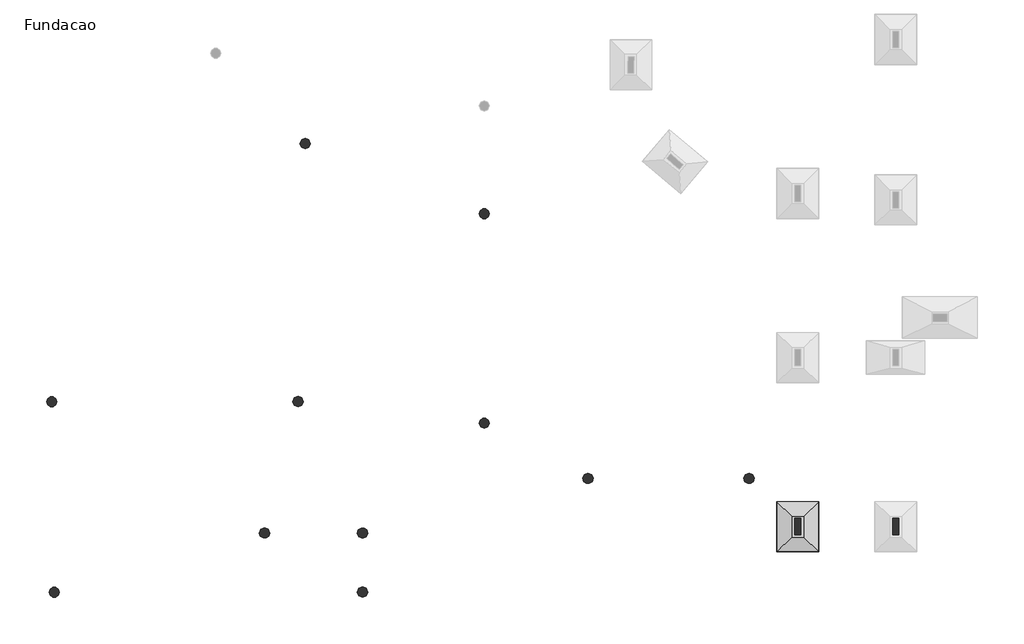
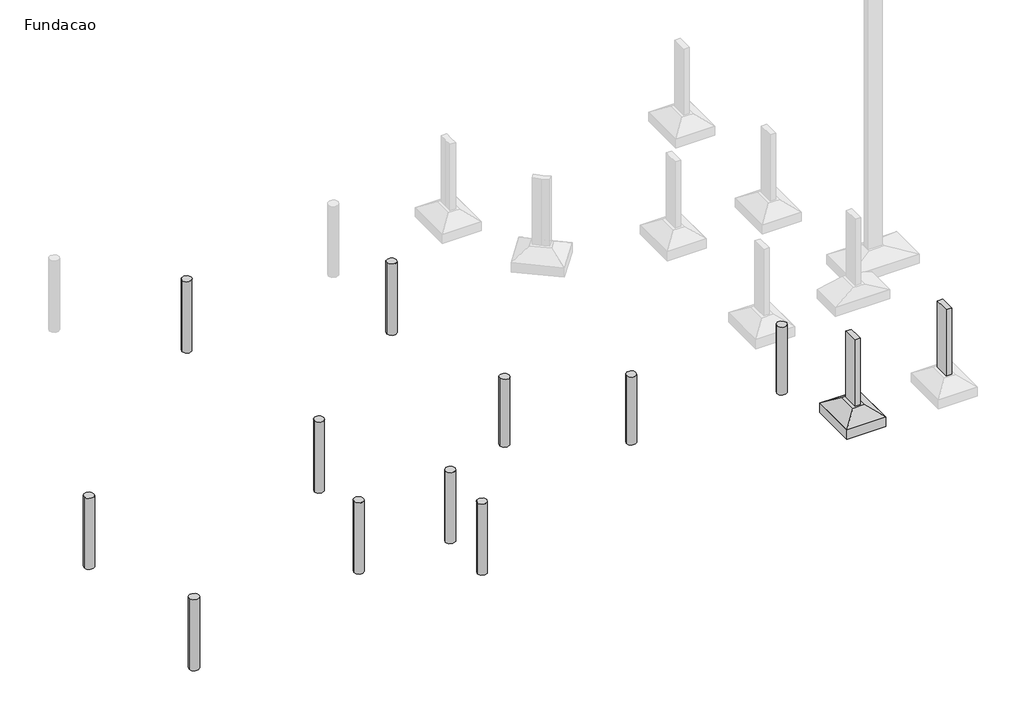
# One storey, part 1 of 2: 13 columns, 1 fastener.
"""IFC4 building model written with IfcOpenShell, lengths in millimetres."""

import ifcopenshell
import ifcopenshell.guid

model = None  # the IFC model being written
_history = None  # IfcOwnerHistory: only IFC2X3 demands one
_inside = {}  # id of a spatial element -> (the spatial element, [elements in it])
_under = {}  # id of a project, library or spatial element -> (it, [spatial elements below it])
_declared = {}  # id of a project -> (the project, [libraries it declares])
_typed = {}  # id of a type object -> (the type object, [elements of that type])
_made_of = {}  # id of a material, layer set ... -> (it, [elements and type objects made of it])


def new_model(schema):
    """Start an empty IFC model of exactly this schema.

    Asked for "IFC4X3", IfcOpenShell would pick the latest addendum, in which some entities
    have other attributes; the version numbers below select the first issue.
    IFC2X3 requires an IfcOwnerHistory on every rooted entity: one is made here for all.
    """
    global model, _history
    if schema == "IFC4X3":
        model = ifcopenshell.file(schema_version=(4, 3, 0, 0))
    else:
        model = ifcopenshell.file(schema=schema)
    _inside.clear()
    _under.clear()
    _declared.clear()
    _typed.clear()
    _made_of.clear()
    _history = None
    if model.schema == "IFC2X3":
        org = make("IfcOrganization", Name="unknown")
        user = make(
            "IfcPersonAndOrganization",
            ThePerson=make("IfcPerson", FamilyName="unknown"),
            TheOrganization=org,
        )
        app = make(
            "IfcApplication",
            ApplicationDeveloper=org,
            Version="unknown",
            ApplicationFullName="unknown",
            ApplicationIdentifier="unknown",
        )
        _history = make(
            "IfcOwnerHistory",
            OwningUser=user,
            OwningApplication=app,
            ChangeAction="ADDED",
            CreationDate=0,
        )
    return model


def make(cls, **values):
    """One entity of the class cls with the attributes given. An attribute that is None is left unset."""
    return model.create_entity(
        cls, **{name: value for name, value in values.items() if value is not None}
    )


def rooted(cls, **values):
    """An entity with a GlobalId (a new one), such as an element, a storey or a relation."""
    return make(cls, GlobalId=ifcopenshell.guid.new(), OwnerHistory=_history, **values)


def si_unit(unit_type, name, prefix=None):
    """IfcSIUnit, for example si_unit("LENGTHUNIT", "METRE", prefix="MILLI")."""
    return make("IfcSIUnit", UnitType=unit_type, Prefix=prefix, Name=name)


def assignment(units):
    """IfcUnitAssignment: the units of a project."""
    return None if units is None else make("IfcUnitAssignment", Units=units)


def point(xyz):
    """IfcCartesianPoint."""
    return None if xyz is None else make("IfcCartesianPoint", Coordinates=xyz)


def direction(xyz):
    """IfcDirection."""
    return None if xyz is None else make("IfcDirection", DirectionRatios=xyz)


def frame(location, z_axis=None, x_axis=None):
    """IfcAxis2Placement3D, a coordinate frame: its origin and axes. An axis left out is left unset."""
    return make(
        "IfcAxis2Placement3D",
        Location=point(location),
        Axis=direction(z_axis),
        RefDirection=direction(x_axis),
    )


def origin():
    """The frame at (0, 0, 0) with its axes left unset."""
    return frame((0.0, 0.0, 0.0))


def place(relative_to, where):
    """IfcLocalPlacement: puts the frame where relative to a parent placement (None: the world)."""
    return make(
        "IfcLocalPlacement", PlacementRelTo=relative_to, RelativePlacement=where
    )


def context(
    kind, dimensions, precision=None, world=None, true_north=None, identifier=None
):
    """IfcGeometricRepresentationContext, for example the 3D "Model" context."""
    return make(
        "IfcGeometricRepresentationContext",
        ContextIdentifier=identifier,
        ContextType=kind,
        CoordinateSpaceDimension=dimensions,
        Precision=precision,
        WorldCoordinateSystem=world,
        TrueNorth=true_north,
    )


def project(units=None, contexts=None):
    """IfcProject with its units and contexts."""
    return rooted(
        "IfcProject",
        Name="project",
        RepresentationContexts=contexts,
        UnitsInContext=assignment(units),
    )


def spatial(cls, under=None, at=None, **own):
    """A site, building, storey or space (cls), placed at a placement, below another one or the project."""
    s = rooted(cls, ObjectPlacement=at, **own)
    if under is not None:
        _under.setdefault(under.id(), (under, []))[1].append(s)
    return s


def polyline(points):
    """IfcPolyline through the points."""
    return make("IfcPolyline", Points=[point(p) for p in points])


def circle_curve(where, radius):
    """IfcCircle in the frame where."""
    return make("IfcCircle", Position=where, Radius=radius)


def outline(outer, holes=None, kind="AREA"):
    """IfcArbitraryClosedProfileDef: a profile drawn as a closed curve; with holes, ...WithVoids."""
    if holes is None:
        return make("IfcArbitraryClosedProfileDef", ProfileType=kind, OuterCurve=outer)
    return make(
        "IfcArbitraryProfileDefWithVoids",
        ProfileType=kind,
        OuterCurve=outer,
        InnerCurves=holes,
    )


def extrude(swept, where, along, depth):
    """IfcExtrudedAreaSolid: the profile swept, set in the frame where, extruded along a direction by depth."""
    return make(
        "IfcExtrudedAreaSolid",
        SweptArea=swept,
        Position=where,
        ExtrudedDirection=direction(along),
        Depth=depth,
    )


def faces_of(points, faces, orient=None, outer=None):
    """IfcFace entities. A face is a list of loops; a loop is a list of indices into points, from 0.

    orient and outer hold one flag for each loop. By default every Orientation is true, the
    first loop of a face is its IfcFaceOuterBound and the others are IfcFaceBound.
    """
    made = []
    for i, loops in enumerate(faces):
        bounds = []
        for j, loop in enumerate(loops):
            is_outer = j == 0 if outer is None else outer[i][j]
            bounds.append(
                make(
                    "IfcFaceOuterBound" if is_outer else "IfcFaceBound",
                    Bound=make("IfcPolyLoop", Polygon=[points[k] for k in loop]),
                    Orientation=True if orient is None else orient[i][j],
                )
            )
        made.append(make("IfcFace", Bounds=bounds))
    return made


def faceted_brep(points, faces, orient=None, outer=None, voids=None):
    """IfcFacetedBrep: a solid bounded by flat faces; with voids (closed shells), ...WithVoids."""
    shared = [point(p) for p in points]
    hull = make("IfcClosedShell", CfsFaces=faces_of(shared, faces, orient, outer))
    if voids is None:
        return make("IfcFacetedBrep", Outer=hull)
    return make(
        "IfcFacetedBrepWithVoids",
        Outer=hull,
        Voids=[
            make(cls, CfsFaces=faces_of(shared, fs, o, b)) for cls, fs, o, b in voids
        ],
    )


def shape(context_of_items, identifier, shape_type, items):
    """IfcShapeRepresentation: the items that make up one representation, for example the "Body"."""
    return make(
        "IfcShapeRepresentation",
        ContextOfItems=context_of_items,
        RepresentationIdentifier=identifier,
        RepresentationType=shape_type,
        Items=items,
    )


def source(mapping_origin, context_of_items, identifier, shape_type, items):
    """IfcRepresentationMap: a shape defined once, which mapped items show again and again."""
    return make(
        "IfcRepresentationMap",
        MappingOrigin=mapping_origin,
        MappedRepresentation=shape(context_of_items, identifier, shape_type, items),
    )


def transform(
    local_origin,
    x_axis=None,
    y_axis=None,
    z_axis=None,
    scale=None,
    scale2=None,
    scale3=None,
    uniform=True,
):
    """IfcCartesianTransformationOperator3D, or its non-uniform kind. x_axis, y_axis, z_axis: its Axis1, 2, 3."""
    if uniform:
        return make(
            "IfcCartesianTransformationOperator3D",
            Axis1=direction(x_axis),
            Axis2=direction(y_axis),
            LocalOrigin=point(local_origin),
            Scale=scale,
            Axis3=direction(z_axis),
        )
    return make(
        "IfcCartesianTransformationOperator3DnonUniform",
        Axis1=direction(x_axis),
        Axis2=direction(y_axis),
        LocalOrigin=point(local_origin),
        Scale=scale,
        Axis3=direction(z_axis),
        Scale2=scale2,
        Scale3=scale3,
    )


def mapped(mapping_source, mapping_target):
    """IfcMappedItem: shows the shape of a source again, moved by a transform."""
    return make(
        "IfcMappedItem", MappingSource=mapping_source, MappingTarget=mapping_target
    )


def made_of(thing, what):
    """Note that an element or type object is made of a material, layer set ...; save() writes the relation."""
    if what is not None:
        _made_of.setdefault(what.id(), (what, []))[1].append(thing)
    return thing


def element(
    cls,
    number,
    at=None,
    inside=None,
    cuts=None,
    type_object=None,
    material=None,
    context=None,
    identifier="Body",
    shape_type=None,
    held_by="IfcProductDefinitionShape",
    body=None,
    shapes=None,
    **own,
):
    """One element of the class cls, such as IfcWall. Its Tag is "e" and its number.

    at: its placement. inside: the storey or other place that contains it. cuts: it is an
    opening in that element (IfcRelVoidsElement). A single representation is given by context,
    identifier, shape_type and body (its items); several are given by shapes. held_by: the class
    of the entity that holds the representations. save() writes the other relations.
    """
    e = rooted(cls, Tag="e%d" % number, ObjectPlacement=at, **own)
    if body is not None:
        shapes = [shape(context, identifier, shape_type, body)]
    if shapes is not None:
        e.Representation = make(held_by, Representations=shapes)
    if inside is not None:
        _inside.setdefault(inside.id(), (inside, []))[1].append(e)
    if cuts is not None:
        rooted(
            "IfcRelVoidsElement", RelatingBuildingElement=cuts, RelatedOpeningElement=e
        )
    if type_object is not None:
        _typed.setdefault(type_object.id(), (type_object, []))[1].append(e)
    return made_of(e, material)


def aggregate(whole, parts):
    """IfcRelAggregates: a whole, such as a stair, and the parts it consists of."""
    return rooted("IfcRelAggregates", RelatingObject=whole, RelatedObjects=parts)


def save(model, path):
    """Write the relations noted so far, then the file.

    IfcRelAggregates (storeys below a building ...), IfcRelContainedInSpatialStructure (elements
    in a storey), IfcRelDefinesByType, IfcRelAssociatesMaterial and IfcRelDeclares: one each for
    every whole, place, type object, material and project.
    """
    for whole, parts in _under.values():
        aggregate(whole, parts)
    for where, things in _inside.values():
        rooted(
            "IfcRelContainedInSpatialStructure",
            RelatedElements=things,
            RelatingStructure=where,
        )
    for kind, things in _typed.values():
        rooted("IfcRelDefinesByType", RelatedObjects=things, RelatingType=kind)
    for what, things in _made_of.values():
        rooted("IfcRelAssociatesMaterial", RelatedObjects=things, RelatingMaterial=what)
    for by, libraries in _declared.values():
        rooted("IfcRelDeclares", RelatingContext=by, RelatedDefinitions=libraries)
    model.write(path)


def plane_surface(at):
    """IfcPlane: the flat surface through the origin of the frame at, square to its z axis."""
    return make("IfcPlane", Position=at)


def cylinder_surface(at, radius):
    """IfcCylindricalSurface: all points at the distance radius from the z axis of the frame at."""
    return make("IfcCylindricalSurface", Position=at, Radius=radius)


def advanced_brep(points, edges, surfaces, faces):
    """IfcAdvancedBrep: a solid bounded by faces that lie on surfaces and meet in shared edges.

    An edge is (start, end): straight between two places in points (the first is 0);
    or (start, end, curve); or (start, end, curve, False) where it runs against its curve.
    A face is (place in surfaces, loops), or (place, loops, False) where it looks against
    its surface's normal. A loop lists edges by number (the first is 1), with a minus sign
    where the edge is run from its end to its start. The first loop is the outer one.
    """
    corners = [point(p) for p in points]
    vertices = [make("IfcVertexPoint", VertexGeometry=c) for c in corners]
    made = []
    for start, end, *more in edges:
        made.append(
            make(
                "IfcEdgeCurve",
                EdgeStart=vertices[start],
                EdgeEnd=vertices[end],
                EdgeGeometry=more[0] if more else make("IfcPolyline", Points=[corners[start], corners[end]]),
                SameSense=more[1] if len(more) > 1 else True,
            )
        )
    hull = []
    for where, loops, *sense in faces:
        bounds = []
        for j, loop in enumerate(loops):
            ring = [make("IfcOrientedEdge", EdgeElement=made[abs(k) - 1], Orientation=k > 0) for k in loop]
            bounds.append(
                make(
                    "IfcFaceOuterBound" if j == 0 else "IfcFaceBound",
                    Bound=make("IfcEdgeLoop", EdgeList=ring),
                    Orientation=True,
                )
            )
        hull.append(make("IfcAdvancedFace", Bounds=bounds, FaceSurface=surfaces[where], SameSense=sense[0] if sense else True))
    return make("IfcAdvancedBrep", Outer=make("IfcClosedShell", CfsFaces=hull))


def sps1_6b3be553(model_context):
    return source(origin(), model_context, "Body", "SolidModel", [
        faceted_brep([(-55.0, 50.0, 0.0), (-345.0, 50.0, 0.0), (-345.0, -450.0, 0.0), (-55.0, -450.0, 0.0), (300.0, 400.0, -250.0), (300.0, -800.0, -250.0), (-700.0, -800.0, -250.0), (-700.0, 400.0, -250.0)], [[[0, 1, 2, 3]], [[4, 5, 6, 7]], [[4, 7, 1, 0]], [[7, 6, 2, 1]], [[6, 5, 3, 2]], [[5, 4, 0, 3]]]),
        extrude(outline(polyline([(300.0, 400.0), (300.0, -800.0), (-700.0, -800.0), (-700.0, 400.0), (300.0, 400.0)])), frame((0.0, 0.0, -500.0), z_axis=(0.0, 0.0, 1.0), x_axis=(1.0, 0.0, 0.0)), (0.0, 0.0, 1.0), 250.0),
    ])


model = new_model("IFC4")

# Units and contexts
model_context = context("Model", 3, world=origin())
ifc_project = project(units=[si_unit("LENGTHUNIT", "METRE", prefix="MILLI")], contexts=[model_context])

# Site, building, storey
site = spatial("IfcSite", under=ifc_project)
building = spatial("IfcBuilding", under=site)
storey = spatial("IfcBuildingStorey", under=building, Name="Fundacao", Elevation=-1200.0)

# Columns
placement = place(None, origin())
element("IfcColumn", 1, ObjectType="TQS - Pilar circular : TQS - Pilar circular 25.0cm", at=placement, inside=storey, context=model_context, shape_type="AdvancedBrep", body=[
    advanced_brep(
    [(-3146.281307, -11048.5699847, -1500.0), (-2896.281307, -11048.5699847, -1500.0), (-3146.281307, -11048.5699847, 430.0), (-3102.521691, -10953.5699847, 430.0), (-2896.281307, -11048.5699847, 430.0), (-3102.521691, -11143.5699847, 430.0)],
    [
        (0, 1, circle_curve(frame((-3021.281307, -11048.5699847, -1500.0), z_axis=(0.0, 0.0, -1.0), x_axis=(1.0, 0.0, 0.0)), 125.0)),
        (1, 0, circle_curve(frame((-3021.281307, -11048.5699847, -1500.0), z_axis=(0.0, 0.0, -1.0), x_axis=(1.0, 0.0, 0.0)), 125.0)),
        (2, 3, circle_curve(frame((-3021.281307, -11048.5699847, 430.0), z_axis=(0.0, 0.0, -1.0), x_axis=(1.0, 0.0, 0.0)), 125.0)),
        (3, 4, circle_curve(frame((-3021.281307, -11048.5699847, 430.0), z_axis=(0.0, 0.0, -1.0), x_axis=(1.0, 0.0, 0.0)), 125.0)),
        (4, 1),
        (0, 2),
        (4, 5, circle_curve(frame((-3021.281307, -11048.5699847, 430.0), z_axis=(0.0, 0.0, -1.0), x_axis=(1.0, 0.0, 0.0)), 125.0)),
        (5, 2, circle_curve(frame((-3021.281307, -11048.5699847, 430.0), z_axis=(0.0, 0.0, -1.0), x_axis=(1.0, 0.0, 0.0)), 125.0)),
    ],
    [
        plane_surface(frame((-2896.281307, -11048.5699847, -1500.0), z_axis=(0.0, 0.0, -1.0), x_axis=(0.0, -1.0, 0.0))),
        cylinder_surface(frame((-3021.281307, -11048.5699847, -1500.0), z_axis=(0.0, 0.0, 1.0), x_axis=(1.0, 0.0, 0.0)), 125.0),
        plane_surface(frame((-2896.281307, -11048.5699847, 430.0), z_axis=(0.0, 0.0, 1.0), x_axis=(0.0, 1.0, 0.0))),
    ],
    [
        (0, [[1, 2]]),
        (1, [[3, 4, 5, -1, 6]]),
        (1, [[7, 8, -6, -2, -5]]),
        (2, [[-8, -7, -4, -3]]),
    ],
),
])
element("IfcColumn", 2, ObjectType="TQS - Pilar circular : TQS - Pilar circular 25.0cm", at=placement, inside=storey, context=model_context, shape_type="AdvancedBrep", body=[
    advanced_brep(
    [(-3146.281307, -9633.3699847, -1500.0), (-2896.281307, -9633.3699847, -1500.0), (-3146.281307, -9633.3699847, 430.0), (-3124.8428828, -9563.3699847, 430.0), (-2896.281307, -9633.3699847, 430.0), (-3124.8428828, -9703.3699847, 430.0)],
    [
        (0, 1, circle_curve(frame((-3021.281307, -9633.3699847, -1500.0), z_axis=(0.0, 0.0, -1.0), x_axis=(1.0, 0.0, 0.0)), 125.0)),
        (1, 0, circle_curve(frame((-3021.281307, -9633.3699847, -1500.0), z_axis=(0.0, 0.0, -1.0), x_axis=(1.0, 0.0, 0.0)), 125.0)),
        (2, 3, circle_curve(frame((-3021.281307, -9633.3699847, 430.0), z_axis=(0.0, 0.0, -1.0), x_axis=(1.0, 0.0, 0.0)), 125.0)),
        (3, 4, circle_curve(frame((-3021.281307, -9633.3699847, 430.0), z_axis=(0.0, 0.0, -1.0), x_axis=(1.0, 0.0, 0.0)), 125.0)),
        (4, 1),
        (0, 2),
        (4, 5, circle_curve(frame((-3021.281307, -9633.3699847, 430.0), z_axis=(0.0, 0.0, -1.0), x_axis=(1.0, 0.0, 0.0)), 125.0)),
        (5, 2, circle_curve(frame((-3021.281307, -9633.3699847, 430.0), z_axis=(0.0, 0.0, -1.0), x_axis=(1.0, 0.0, 0.0)), 125.0)),
    ],
    [
        plane_surface(frame((-2896.281307, -9633.3699847, -1500.0), z_axis=(0.0, 0.0, -1.0), x_axis=(0.0, -1.0, 0.0))),
        cylinder_surface(frame((-3021.281307, -9633.3699847, -1500.0), z_axis=(0.0, 0.0, 1.0), x_axis=(1.0, 0.0, 0.0)), 125.0),
        plane_surface(frame((-2896.281307, -9633.3699847, 430.0), z_axis=(0.0, 0.0, 1.0), x_axis=(0.0, 1.0, 0.0))),
    ],
    [
        (0, [[1, 2]]),
        (1, [[3, 4, 5, -1, 6]]),
        (1, [[7, 8, -6, -2, -5]]),
        (2, [[-8, -7, -4, -3]]),
    ],
),
])
element("IfcColumn", 3, ObjectType="TQS - Pilar circular : TQS - Pilar circular 25.0cm", at=placement, inside=storey, context=model_context, shape_type="AdvancedBrep", body=[
    advanced_brep(
    [(-10536.281307, -11048.5699847, -1500.0), (-10286.281307, -11048.5699847, -1500.0), (-10536.281307, -11048.5699847, 430.0), (-10492.499945, -10953.5513927, 430.0), (-10401.3039585, -10923.9688109, 430.0), (-10330.0409229, -10953.5699847, 430.0), (-10286.281307, -11048.5699847, 430.0), (-10330.0409229, -11143.5699847, 430.0), (-10492.499945, -11143.5885767, 430.0)],
    [
        (0, 1, circle_curve(frame((-10411.281307, -11048.5699847, -1500.0), z_axis=(0.0, 0.0, -1.0), x_axis=(1.0, 0.0, 0.0)), 125.0)),
        (1, 0, circle_curve(frame((-10411.281307, -11048.5699847, -1500.0), z_axis=(0.0, 0.0, -1.0), x_axis=(1.0, 0.0, 0.0)), 125.0)),
        (2, 3, circle_curve(frame((-10411.281307, -11048.5699847, 430.0), z_axis=(0.0, 0.0, -1.0), x_axis=(1.0, 0.0, 0.0)), 125.0)),
        (3, 4, circle_curve(frame((-10411.281307, -11048.5699847, 430.0), z_axis=(0.0, 0.0, -1.0), x_axis=(1.0, 0.0, 0.0)), 125.0)),
        (4, 5, circle_curve(frame((-10411.281307, -11048.5699847, 430.0), z_axis=(0.0, 0.0, -1.0), x_axis=(1.0, 0.0, 0.0)), 125.0)),
        (5, 6, circle_curve(frame((-10411.281307, -11048.5699847, 430.0), z_axis=(0.0, 0.0, -1.0), x_axis=(1.0, 0.0, 0.0)), 125.0)),
        (6, 1),
        (0, 2),
        (6, 7, circle_curve(frame((-10411.281307, -11048.5699847, 430.0), z_axis=(0.0, 0.0, -1.0), x_axis=(1.0, 0.0, 0.0)), 125.0)),
        (7, 8, circle_curve(frame((-10411.281307, -11048.5699847, 430.0), z_axis=(0.0, 0.0, -1.0), x_axis=(1.0, 0.0, 0.0)), 125.0)),
        (8, 2, circle_curve(frame((-10411.281307, -11048.5699847, 430.0), z_axis=(0.0, 0.0, -1.0), x_axis=(1.0, 0.0, 0.0)), 125.0)),
    ],
    [
        plane_surface(frame((-10286.281307, -11048.5699847, -1500.0), z_axis=(0.0, 0.0, -1.0), x_axis=(0.0, -1.0, 0.0))),
        cylinder_surface(frame((-10411.281307, -11048.5699847, -1500.0), z_axis=(0.0, 0.0, 1.0), x_axis=(1.0, 0.0, 0.0)), 125.0),
        plane_surface(frame((-10286.281307, -11048.5699847, 430.0), z_axis=(0.0, 0.0, 1.0), x_axis=(0.0, 1.0, 0.0))),
    ],
    [
        (0, [[1, 2]]),
        (1, [[3, 4, 5, 6, 7, -1, 8]]),
        (1, [[9, 10, 11, -8, -2, -7]]),
        (2, [[-11, -10, -9, -6, -5, -4, -3]]),
    ],
),
])
element("IfcColumn", 4, ObjectType="TQS - Pilar circular : TQS - Pilar circular 25.0cm", at=placement, inside=storey, context=model_context, shape_type="AdvancedBrep", body=[
    advanced_brep(
    [(-4522.481307, -299.9062997, -1500.0), (-4272.481307, -299.9062997, -1500.0), (-4522.481307, -299.9062997, 430.0), (-4272.481307, -299.9062997, 430.0), (-4327.481307, -403.4678755, 430.0), (-4467.481307, -403.4678755, 430.0)],
    [
        (0, 1, circle_curve(frame((-4397.481307, -299.9062997, -1500.0), z_axis=(0.0, 0.0, -1.0), x_axis=(1.0, 0.0, 0.0)), 125.0)),
        (1, 0, circle_curve(frame((-4397.481307, -299.9062997, -1500.0), z_axis=(0.0, 0.0, -1.0), x_axis=(1.0, 0.0, 0.0)), 125.0)),
        (2, 3, circle_curve(frame((-4397.481307, -299.9062997, 430.0), z_axis=(0.0, 0.0, -1.0), x_axis=(1.0, 0.0, 0.0)), 125.0)),
        (3, 1),
        (0, 2),
        (3, 4, circle_curve(frame((-4397.481307, -299.9062997, 430.0), z_axis=(0.0, 0.0, -1.0), x_axis=(1.0, 0.0, 0.0)), 125.0)),
        (4, 5, circle_curve(frame((-4397.481307, -299.9062997, 430.0), z_axis=(0.0, 0.0, -1.0), x_axis=(1.0, 0.0, 0.0)), 125.0)),
        (5, 2, circle_curve(frame((-4397.481307, -299.9062997, 430.0), z_axis=(0.0, 0.0, -1.0), x_axis=(1.0, 0.0, 0.0)), 125.0)),
    ],
    [
        plane_surface(frame((-4272.481307, -299.9062997, -1500.0), z_axis=(0.0, 0.0, -1.0), x_axis=(0.0, -1.0, 0.0))),
        cylinder_surface(frame((-4397.481307, -299.9062997, -1500.0), z_axis=(0.0, 0.0, 1.0), x_axis=(1.0, 0.0, 0.0)), 125.0),
        plane_surface(frame((-4272.481307, -299.9062997, 430.0), z_axis=(0.0, 0.0, 1.0), x_axis=(0.0, 1.0, 0.0))),
    ],
    [
        (0, [[1, 2]]),
        (1, [[3, 4, -1, 5]]),
        (1, [[6, 7, 8, -5, -2, -4]]),
        (2, [[-8, -7, -6, -3]]),
    ],
),
])
element("IfcColumn", 5, ObjectType="TQS - Pilar circular : TQS - Pilar circular 25.0cm", at=placement, inside=storey, context=model_context, shape_type="AdvancedBrep", body=[
    advanced_brep(
    [(-232.281307, -1983.5699847, -1500.0), (17.718693, -1983.5699847, -1500.0), (-232.281307, -1983.5699847, 430.0), (-202.281307, -1902.3296007, 430.0), (-12.281307, -1902.3296007, 430.0), (17.718693, -1983.5699847, 430.0), (-12.281307, -2064.8103688, 430.0), (-202.281307, -2064.8103688, 430.0)],
    [
        (0, 1, circle_curve(frame((-107.281307, -1983.5699847, -1500.0), z_axis=(0.0, 0.0, -1.0), x_axis=(1.0, 0.0, 0.0)), 125.0)),
        (1, 0, circle_curve(frame((-107.281307, -1983.5699847, -1500.0), z_axis=(0.0, 0.0, -1.0), x_axis=(1.0, 0.0, 0.0)), 125.0)),
        (2, 3, circle_curve(frame((-107.281307, -1983.5699847, 430.0), z_axis=(0.0, 0.0, -1.0), x_axis=(1.0, 0.0, 0.0)), 125.0)),
        (3, 4, circle_curve(frame((-107.281307, -1983.5699847, 430.0), z_axis=(0.0, 0.0, -1.0), x_axis=(1.0, 0.0, 0.0)), 125.0)),
        (4, 5, circle_curve(frame((-107.281307, -1983.5699847, 430.0), z_axis=(0.0, 0.0, -1.0), x_axis=(1.0, 0.0, 0.0)), 125.0)),
        (5, 1),
        (0, 2),
        (5, 6, circle_curve(frame((-107.281307, -1983.5699847, 430.0), z_axis=(0.0, 0.0, -1.0), x_axis=(1.0, 0.0, 0.0)), 125.0)),
        (6, 7, circle_curve(frame((-107.281307, -1983.5699847, 430.0), z_axis=(0.0, 0.0, -1.0), x_axis=(1.0, 0.0, 0.0)), 125.0)),
        (7, 2, circle_curve(frame((-107.281307, -1983.5699847, 430.0), z_axis=(0.0, 0.0, -1.0), x_axis=(1.0, 0.0, 0.0)), 125.0)),
    ],
    [
        plane_surface(frame((17.718693, -1983.5699847, -1500.0), z_axis=(0.0, 0.0, -1.0), x_axis=(0.0, -1.0, 0.0))),
        cylinder_surface(frame((-107.281307, -1983.5699847, -1500.0), z_axis=(0.0, 0.0, 1.0), x_axis=(1.0, 0.0, 0.0)), 125.0),
        plane_surface(frame((17.718693, -1983.5699847, 430.0), z_axis=(0.0, 0.0, 1.0), x_axis=(0.0, 1.0, 0.0))),
    ],
    [
        (0, [[1, 2]]),
        (1, [[3, 4, 5, 6, -1, 7]]),
        (1, [[8, 9, 10, -7, -2, -6]]),
        (2, [[-10, -9, -8, -5, -4, -3]]),
    ],
),
])
element("IfcColumn", 6, ObjectType="TQS - Pilar circular : TQS - Pilar circular 25.0cm", at=placement, inside=storey, context=model_context, shape_type="AdvancedBrep", body=[
    advanced_brep(
    [(-232.281307, -7001.4699847, -1500.0), (17.718693, -7001.4699847, -1500.0), (-232.281307, -7001.4699847, 340.0), (-202.281307, -6920.2296007, 340.0), (-12.281307, -6920.2296007, 340.0), (17.718693, -7001.4699847, 340.0), (-12.281307, -7082.7103687, 340.0), (-202.281307, -7082.7103687, 340.0)],
    [
        (0, 1, circle_curve(frame((-107.281307, -7001.4699847, -1500.0), z_axis=(0.0, 0.0, -1.0), x_axis=(1.0, 0.0, 0.0)), 125.0)),
        (1, 0, circle_curve(frame((-107.281307, -7001.4699847, -1500.0), z_axis=(0.0, 0.0, -1.0), x_axis=(1.0, 0.0, 0.0)), 125.0)),
        (2, 3, circle_curve(frame((-107.281307, -7001.4699847, 340.0), z_axis=(0.0, 0.0, -1.0), x_axis=(1.0, 0.0, 0.0)), 125.0)),
        (3, 4, circle_curve(frame((-107.281307, -7001.4699847, 340.0), z_axis=(0.0, 0.0, -1.0), x_axis=(1.0, 0.0, 0.0)), 125.0)),
        (4, 5, circle_curve(frame((-107.281307, -7001.4699847, 340.0), z_axis=(0.0, 0.0, -1.0), x_axis=(1.0, 0.0, 0.0)), 125.0)),
        (5, 1),
        (0, 2),
        (5, 6, circle_curve(frame((-107.281307, -7001.4699847, 340.0), z_axis=(0.0, 0.0, -1.0), x_axis=(1.0, 0.0, 0.0)), 125.0)),
        (6, 7, circle_curve(frame((-107.281307, -7001.4699847, 340.0), z_axis=(0.0, 0.0, -1.0), x_axis=(1.0, 0.0, 0.0)), 125.0)),
        (7, 2, circle_curve(frame((-107.281307, -7001.4699847, 340.0), z_axis=(0.0, 0.0, -1.0), x_axis=(1.0, 0.0, 0.0)), 125.0)),
    ],
    [
        plane_surface(frame((17.718693, -7001.4699847, -1500.0), z_axis=(0.0, 0.0, -1.0), x_axis=(0.0, -1.0, 0.0))),
        cylinder_surface(frame((-107.281307, -7001.4699847, -1500.0), z_axis=(0.0, 0.0, 1.0), x_axis=(1.0, 0.0, 0.0)), 125.0),
        plane_surface(frame((17.718693, -7001.4699847, 340.0), z_axis=(0.0, 0.0, 1.0), x_axis=(0.0, 1.0, 0.0))),
    ],
    [
        (0, [[1, 2]]),
        (1, [[3, 4, 5, 6, -1, 7]]),
        (1, [[8, 9, 10, -7, -2, -6]]),
        (2, [[-10, -9, -8, -5, -4, -3]]),
    ],
),
])
element("IfcColumn", 7, ObjectType="TQS - Pilar circular : TQS - Pilar circular 25.0cm", at=placement, inside=storey, context=model_context, shape_type="AdvancedBrep", body=[
    advanced_brep(
    [(-10596.281307, -6483.3699847, -1500.0), (-10346.281307, -6483.3699847, -1500.0), (-10596.281307, -6483.3699847, 430.0), (-10574.8428829, -6413.3699847, 430.0), (-10541.2456335, -6379.7843051, 430.0), (-10401.2667974, -6379.8182177, 430.0), (-10367.7370456, -6413.3443756, 430.0), (-10346.281307, -6483.3699847, 430.0), (-10367.7370456, -6553.3955938, 430.0), (-10401.2667974, -6586.9217517, 430.0), (-10541.2456335, -6586.9556643, 430.0), (-10574.8428829, -6553.3699847, 430.0)],
    [
        (0, 1, circle_curve(frame((-10471.281307, -6483.3699847, -1500.0), z_axis=(0.0, 0.0, -1.0), x_axis=(1.0, 0.0, 0.0)), 125.0)),
        (1, 0, circle_curve(frame((-10471.281307, -6483.3699847, -1500.0), z_axis=(0.0, 0.0, -1.0), x_axis=(1.0, 0.0, 0.0)), 125.0)),
        (2, 3, circle_curve(frame((-10471.281307, -6483.3699847, 430.0), z_axis=(0.0, 0.0, -1.0), x_axis=(1.0, 0.0, 0.0)), 125.0)),
        (3, 4, circle_curve(frame((-10471.281307, -6483.3699847, 430.0), z_axis=(0.0, 0.0, -1.0), x_axis=(1.0, 0.0, 0.0)), 125.0)),
        (4, 5, circle_curve(frame((-10471.281307, -6483.3699847, 430.0), z_axis=(0.0, 0.0, -1.0), x_axis=(1.0, 0.0, 0.0)), 125.0)),
        (5, 6, circle_curve(frame((-10471.281307, -6483.3699847, 430.0), z_axis=(0.0, 0.0, -1.0), x_axis=(1.0, 0.0, 0.0)), 125.0)),
        (6, 7, circle_curve(frame((-10471.281307, -6483.3699847, 430.0), z_axis=(0.0, 0.0, -1.0), x_axis=(1.0, 0.0, 0.0)), 125.0)),
        (7, 1),
        (0, 2),
        (7, 8, circle_curve(frame((-10471.281307, -6483.3699847, 430.0), z_axis=(0.0, 0.0, -1.0), x_axis=(1.0, 0.0, 0.0)), 125.0)),
        (8, 9, circle_curve(frame((-10471.281307, -6483.3699847, 430.0), z_axis=(0.0, 0.0, -1.0), x_axis=(1.0, 0.0, 0.0)), 125.0)),
        (9, 10, circle_curve(frame((-10471.281307, -6483.3699847, 430.0), z_axis=(0.0, 0.0, -1.0), x_axis=(1.0, 0.0, 0.0)), 125.0)),
        (10, 11, circle_curve(frame((-10471.281307, -6483.3699847, 430.0), z_axis=(0.0, 0.0, -1.0), x_axis=(1.0, 0.0, 0.0)), 125.0)),
        (11, 2, circle_curve(frame((-10471.281307, -6483.3699847, 430.0), z_axis=(0.0, 0.0, -1.0), x_axis=(1.0, 0.0, 0.0)), 125.0)),
    ],
    [
        plane_surface(frame((-10346.281307, -6483.3699847, -1500.0), z_axis=(0.0, 0.0, -1.0), x_axis=(0.0, -1.0, 0.0))),
        cylinder_surface(frame((-10471.281307, -6483.3699847, -1500.0), z_axis=(0.0, 0.0, 1.0), x_axis=(1.0, 0.0, 0.0)), 125.0),
        plane_surface(frame((-10346.281307, -6483.3699847, 430.0), z_axis=(0.0, 0.0, 1.0), x_axis=(0.0, 1.0, 0.0))),
    ],
    [
        (0, [[1, 2]]),
        (1, [[3, 4, 5, 6, 7, 8, -1, 9]]),
        (1, [[10, 11, 12, 13, 14, -9, -2, -8]]),
        (2, [[-14, -13, -12, -11, -10, -7, -6, -5, -4, -3]]),
    ],
),
])
element("IfcColumn", 8, ObjectType="TQS - Pilar circular : TQS - Pilar circular 25.0cm", at=placement, inside=storey, context=model_context, shape_type="AdvancedBrep", body=[
    advanced_brep(
    [(-4691.281307, -6483.3699847, -1500.0), (-4441.281307, -6483.3699847, -1500.0), (-4691.281307, -6483.3699847, 430.0), (-4669.8428828, -6413.3699847, 430.0), (-4611.2575682, -6366.7417895, 430.0), (-4471.3008134, -6402.106796, 430.0), (-4441.281307, -6483.3699847, 430.0), (-4669.8428828, -6553.3699847, 430.0)],
    [
        (0, 1, circle_curve(frame((-4566.281307, -6483.3699847, -1500.0), z_axis=(0.0, 0.0, -1.0), x_axis=(1.0, 0.0, 0.0)), 125.0)),
        (1, 0, circle_curve(frame((-4566.281307, -6483.3699847, -1500.0), z_axis=(0.0, 0.0, -1.0), x_axis=(1.0, 0.0, 0.0)), 125.0)),
        (2, 3, circle_curve(frame((-4566.281307, -6483.3699847, 430.0), z_axis=(0.0, 0.0, -1.0), x_axis=(1.0, 0.0, 0.0)), 125.0)),
        (3, 4, circle_curve(frame((-4566.281307, -6483.3699847, 430.0), z_axis=(0.0, 0.0, -1.0), x_axis=(1.0, 0.0, 0.0)), 125.0)),
        (4, 5, circle_curve(frame((-4566.281307, -6483.3699847, 430.0), z_axis=(0.0, 0.0, -1.0), x_axis=(1.0, 0.0, 0.0)), 125.0)),
        (5, 6, circle_curve(frame((-4566.281307, -6483.3699847, 430.0), z_axis=(0.0, 0.0, -1.0), x_axis=(1.0, 0.0, 0.0)), 125.0)),
        (6, 1),
        (0, 2),
        (6, 7, circle_curve(frame((-4566.281307, -6483.3699847, 430.0), z_axis=(0.0, 0.0, -1.0), x_axis=(1.0, 0.0, 0.0)), 125.0)),
        (7, 2, circle_curve(frame((-4566.281307, -6483.3699847, 430.0), z_axis=(0.0, 0.0, -1.0), x_axis=(1.0, 0.0, 0.0)), 125.0)),
    ],
    [
        plane_surface(frame((-4441.281307, -6483.3699847, -1500.0), z_axis=(0.0, 0.0, -1.0), x_axis=(0.0, -1.0, 0.0))),
        cylinder_surface(frame((-4566.281307, -6483.3699847, -1500.0), z_axis=(0.0, 0.0, 1.0), x_axis=(1.0, 0.0, 0.0)), 125.0),
        plane_surface(frame((-4441.281307, -6483.3699847, 430.0), z_axis=(0.0, 0.0, 1.0), x_axis=(0.0, 1.0, 0.0))),
    ],
    [
        (0, [[1, 2]]),
        (1, [[3, 4, 5, 6, 7, -1, 8]]),
        (1, [[9, 10, -8, -2, -7]]),
        (2, [[-10, -9, -6, -5, -4, -3]]),
    ],
),
])
element("IfcColumn", 9, ObjectType="TQS - Pilar circular : TQS - Pilar circular 25.0cm", at=placement, inside=storey, context=model_context, shape_type="AdvancedBrep", body=[
    advanced_brep(
    [(2251.718693, -8326.6699847, -1500.0), (2501.718693, -8326.6699847, -1500.0), (2251.718693, -8326.6699847, 340.0), (2480.2802689, -8256.6699847, 340.0), (2501.718693, -8326.6699847, 340.0), (2480.2802689, -8396.6699847, 340.0)],
    [
        (0, 1, circle_curve(frame((2376.718693, -8326.6699847, -1500.0), z_axis=(0.0, 0.0, -1.0), x_axis=(1.0, 0.0, 0.0)), 125.0)),
        (1, 0, circle_curve(frame((2376.718693, -8326.6699847, -1500.0), z_axis=(0.0, 0.0, -1.0), x_axis=(1.0, 0.0, 0.0)), 125.0)),
        (2, 3, circle_curve(frame((2376.718693, -8326.6699847, 340.0), z_axis=(0.0, 0.0, -1.0), x_axis=(1.0, 0.0, 0.0)), 125.0)),
        (3, 4, circle_curve(frame((2376.718693, -8326.6699847, 340.0), z_axis=(0.0, 0.0, -1.0), x_axis=(1.0, 0.0, 0.0)), 125.0)),
        (4, 1),
        (0, 2),
        (4, 5, circle_curve(frame((2376.718693, -8326.6699847, 340.0), z_axis=(0.0, 0.0, -1.0), x_axis=(1.0, 0.0, 0.0)), 125.0)),
        (5, 2, circle_curve(frame((2376.718693, -8326.6699847, 340.0), z_axis=(0.0, 0.0, -1.0), x_axis=(1.0, 0.0, 0.0)), 125.0)),
    ],
    [
        plane_surface(frame((2501.718693, -8326.6699847, -1500.0), z_axis=(0.0, 0.0, -1.0), x_axis=(0.0, -1.0, 0.0))),
        cylinder_surface(frame((2376.718693, -8326.6699847, -1500.0), z_axis=(0.0, 0.0, 1.0), x_axis=(1.0, 0.0, 0.0)), 125.0),
        plane_surface(frame((2501.718693, -8326.6699847, 340.0), z_axis=(0.0, 0.0, 1.0), x_axis=(0.0, 1.0, 0.0))),
    ],
    [
        (0, [[1, 2]]),
        (1, [[3, 4, 5, -1, 6]]),
        (1, [[7, 8, -6, -2, -5]]),
        (2, [[-8, -7, -4, -3]]),
    ],
),
])
element("IfcColumn", 10, ObjectType="TQS - Pilar circular : TQS - Pilar circular 25.0cm", at=placement, inside=storey, context=model_context, shape_type="AdvancedBrep", body=[
    advanced_brep(
    [(6115.718693, -8326.6699847, -1500.0), (6365.718693, -8326.6699847, -1500.0), (6115.718693, -8326.6699847, 340.0), (6137.1571171, -8256.6699847, 340.0), (6365.718693, -8326.6699847, 340.0), (6137.1571171, -8396.6699847, 340.0)],
    [
        (0, 1, circle_curve(frame((6240.718693, -8326.6699847, -1500.0), z_axis=(0.0, 0.0, -1.0), x_axis=(1.0, 0.0, 0.0)), 125.0)),
        (1, 0, circle_curve(frame((6240.718693, -8326.6699847, -1500.0), z_axis=(0.0, 0.0, -1.0), x_axis=(1.0, 0.0, 0.0)), 125.0)),
        (2, 3, circle_curve(frame((6240.718693, -8326.6699847, 340.0), z_axis=(0.0, 0.0, -1.0), x_axis=(1.0, 0.0, 0.0)), 125.0)),
        (3, 4, circle_curve(frame((6240.718693, -8326.6699847, 340.0), z_axis=(0.0, 0.0, -1.0), x_axis=(1.0, 0.0, 0.0)), 125.0)),
        (4, 1),
        (0, 2),
        (4, 5, circle_curve(frame((6240.718693, -8326.6699847, 340.0), z_axis=(0.0, 0.0, -1.0), x_axis=(1.0, 0.0, 0.0)), 125.0)),
        (5, 2, circle_curve(frame((6240.718693, -8326.6699847, 340.0), z_axis=(0.0, 0.0, -1.0), x_axis=(1.0, 0.0, 0.0)), 125.0)),
    ],
    [
        plane_surface(frame((6365.718693, -8326.6699847, -1500.0), z_axis=(0.0, 0.0, -1.0), x_axis=(0.0, -1.0, 0.0))),
        cylinder_surface(frame((6240.718693, -8326.6699847, -1500.0), z_axis=(0.0, 0.0, 1.0), x_axis=(1.0, 0.0, 0.0)), 125.0),
        plane_surface(frame((6365.718693, -8326.6699847, 340.0), z_axis=(0.0, 0.0, 1.0), x_axis=(0.0, 1.0, 0.0))),
    ],
    [
        (0, [[1, 2]]),
        (1, [[3, 4, 5, -1, 6]]),
        (1, [[7, 8, -6, -2, -5]]),
        (2, [[-8, -7, -4, -3]]),
    ],
),
])
element("IfcColumn", 11, ObjectType="TQS - Pilar circular : TQS - Pilar circular 25.0cm", at=placement, inside=storey, context=model_context, shape_type="AdvancedBrep", body=[
    advanced_brep(
    [(-5495.081307, -9633.3699847, -1500.0), (-5245.081307, -9633.3699847, -1500.0), (-5495.081307, -9633.3699847, 430.0), (-5440.081307, -9529.8084088, 430.0), (-5300.081307, -9529.8084088, 430.0), (-5266.5138113, -9563.3787435, 430.0), (-5245.081307, -9633.3699847, 430.0), (-5266.5138113, -9703.3612259, 430.0), (-5300.081307, -9736.9315606, 430.0), (-5440.081307, -9736.9315606, 430.0)],
    [
        (0, 1, circle_curve(frame((-5370.081307, -9633.3699847, -1500.0), z_axis=(0.0, 0.0, -1.0), x_axis=(1.0, 0.0, 0.0)), 125.0)),
        (1, 0, circle_curve(frame((-5370.081307, -9633.3699847, -1500.0), z_axis=(0.0, 0.0, -1.0), x_axis=(1.0, 0.0, 0.0)), 125.0)),
        (2, 3, circle_curve(frame((-5370.081307, -9633.3699847, 430.0), z_axis=(0.0, 0.0, -1.0), x_axis=(1.0, 0.0, 0.0)), 125.0)),
        (3, 4, circle_curve(frame((-5370.081307, -9633.3699847, 430.0), z_axis=(0.0, 0.0, -1.0), x_axis=(1.0, 0.0, 0.0)), 125.0)),
        (4, 5, circle_curve(frame((-5370.081307, -9633.3699847, 430.0), z_axis=(0.0, 0.0, -1.0), x_axis=(1.0, 0.0, 0.0)), 125.0)),
        (5, 6, circle_curve(frame((-5370.081307, -9633.3699847, 430.0), z_axis=(0.0, 0.0, -1.0), x_axis=(1.0, 0.0, 0.0)), 125.0)),
        (6, 1),
        (0, 2),
        (6, 7, circle_curve(frame((-5370.081307, -9633.3699847, 430.0), z_axis=(0.0, 0.0, -1.0), x_axis=(1.0, 0.0, 0.0)), 125.0)),
        (7, 8, circle_curve(frame((-5370.081307, -9633.3699847, 430.0), z_axis=(0.0, 0.0, -1.0), x_axis=(1.0, 0.0, 0.0)), 125.0)),
        (8, 9, circle_curve(frame((-5370.081307, -9633.3699847, 430.0), z_axis=(0.0, 0.0, -1.0), x_axis=(1.0, 0.0, 0.0)), 125.0)),
        (9, 2, circle_curve(frame((-5370.081307, -9633.3699847, 430.0), z_axis=(0.0, 0.0, -1.0), x_axis=(1.0, 0.0, 0.0)), 125.0)),
    ],
    [
        plane_surface(frame((-5245.081307, -9633.3699847, -1500.0), z_axis=(0.0, 0.0, -1.0), x_axis=(0.0, -1.0, 0.0))),
        cylinder_surface(frame((-5370.081307, -9633.3699847, -1500.0), z_axis=(0.0, 0.0, 1.0), x_axis=(1.0, 0.0, 0.0)), 125.0),
        plane_surface(frame((-5245.081307, -9633.3699847, 430.0), z_axis=(0.0, 0.0, 1.0), x_axis=(0.0, 1.0, 0.0))),
    ],
    [
        (0, [[1, 2]]),
        (1, [[3, 4, 5, 6, 7, -1, 8]]),
        (1, [[9, 10, 11, 12, -8, -2, -7]]),
        (2, [[-12, -11, -10, -9, -6, -5, -4, -3]]),
    ],
),
])
element("IfcColumn", 12, ObjectType="TQS - Pilar retangular : 14.0 x 40.0", at=placement, inside=storey, context=model_context, shape_type="Brep", body=[
    faceted_brep([(7334.718693, -9679.5699847, -1450.0), (7334.718693, -9279.5699847, -1450.0), (7474.718693, -9279.5699847, -1450.0), (7474.718693, -9539.5699847, -1450.0), (7474.718693, -9679.5699847, -1450.0), (7334.718693, -9679.5699847, 350.0), (7334.718693, -9279.5699847, 350.0), (7474.718693, -9279.5699847, 350.0), (7474.718693, -9279.5699847, -1250.0), (7474.718693, -9539.5699847, 350.0), (7474.718693, -9679.5699847, 350.0)], [[[0, 1, 2, 3, 4]], [[1, 0, 5, 6]], [[2, 1, 6, 7, 8]], [[7, 9, 10, 4, 3, 2, 8]], [[0, 4, 10, 5]], [[6, 5, 10, 9, 7]]]),
])
element("IfcColumn", 13, ObjectType="TQS - Pilar retangular : 14.0 x 40.0", at=placement, inside=storey, context=model_context, shape_type="Brep", body=[
    faceted_brep([(9682.718693, -9679.5699847, -1450.0), (9682.718693, -9539.5699847, -1450.0), (9682.718693, -9279.5699847, -1450.0), (9822.718693, -9279.5699847, -1450.0), (9822.718693, -9679.5699847, -1450.0), (9682.718693, -9679.5699847, 350.0), (9682.718693, -9539.5699847, 350.0), (9682.718693, -9279.5699847, 350.0), (9822.718693, -9279.5699847, 350.0), (9822.718693, -9679.5699847, 350.0)], [[[0, 1, 2, 3, 4]], [[5, 6, 7, 2, 1, 0]], [[7, 8, 3, 2]], [[8, 9, 4, 3]], [[9, 5, 0, 4]], [[5, 9, 8, 7, 6]]]),
])

# Fastener
sps1_shape = sps1_6b3be553(model_context)
element("IfcFastener", 14, ObjectType="TQS - Sapata : SPS9", at=placement, inside=storey, context=model_context, shape_type="MappedRepresentation", body=[
    mapped(sps1_shape, transform((7604.718693, -9279.5699847, -1450.0), x_axis=(1.0, 0.0, 0.0), y_axis=(0.0, 1.0, 0.0), z_axis=(0.0, 0.0, 1.0))),
])

save(model, "model.ifc")

# Revit data of these elements
# Project information
#   Design Option = "Main Model"
#   Project Status = "Status do projeto"
#   Project Address = "RUA SÉRGIO DIAS, LOTE 30, QUADRA G, MONTE MINEIRO/MG"
#   Project Name = "RESIDÊNCIA - ROBERTA VENDRAMINI"
#   Project Number = "034/2017"
#   Zona = "ZER - 01"
#   CA Mín = "0.2"
#   CA Básico = "1"
#   CA Máx = "2"
#   TO Máx = "50"
#   Gabarito Máx = "10"
#   TP Mín = "15"
#   Área Total do Terreno = "620.00 m²"
#   Multifamiliar - Vagas Veículos/Pavto = "0"
#   Multifamiliar - Vagas Bicicletas/Pavto = "0"
#   Multifamiliar - % Vagas PNMR = "0"
#   Multifamiliar - % Vagas Motos = "0"
#   Outros - Área p/ 1 Veículo = "0.00 m²"
#   Outros - Área p/ 1 Bicicleta = "0.00 m²"
#   Outros - Área p/ 1 Utilitário = "0.00 m²"
#   Outros - % Vagas PNMR = "0"
#   Outros - % Vagas Motos = "0"
# Type "TQS - Pilar circular : TQS - Pilar circular 25.0cm"
#   b = 0.25 m
#   Structural Material [instance default] = Concrete - Cast-in-Place Concrete
# Type "TQS - Pilar retangular : 14.0 x 40.0"
#   b = 0.14 m
#   h = 0.40 m
#   Structural Material [instance default] = Concrete - Cast-in-Place Concrete
# Type "TQS - Sapata : SPS9"
#   TY = 0.50 m
#   TX = 0.29 m
#   HS = 0.50 m
#   H0 = 0.25 m
#   EXCYABS = 0.60 m
#   EXCY = 0.00 m
#   EXCXABS = 0.50 m
#   EXCX = 0.00 m
#   DIMY = 1.20 m
#   DIMX = 1.00 m
#   Material estrutural = Concreto - Concreto concretado no local
#   Width = 0
#   Length = 0
# Element 1 (IfcColumn, "TQS - Pilar circular : TQS - Pilar circular 25.0cm")
#   Uso = "ESTRUTURA"
#   Titulo = "B16"
#   Chave = "B16//0"
#   Tipo Elemento = "Pilar"
#   SHA1 = "82B48CD5E8973EF4D0B8CB7C6B44CDDBAEC6BB1B"
#   Revisão = ""
#   Tipo de carga = ""
#   Divisor de flexao = ""
#   Secao = "C 25"
#   Configuracao = ""
#   Angulo (graus) = ""
#   Detalhamento = ""
#   Casos de vento manual = ""
#   Tipo = ""
#   Alcas = ""
#   Furos = ""
#   Pino = ""
#   Distribuicao = ""
#   Solidarizado = ""
#   Solidarizar na montagem = ""
#   Unir com o próximo = ""
#   Grupo pre moldado = ""
#   Verificado = ""
#   Concreto C = ""
#   Taxa de armadura (kgf/m³) = 0
#   Carga (tf/m²) = 0
#   Carga (tf/m) = 0
#   Carga (tf) = 0
#   Altura = 1.70 m
#   Rebaixo = 0.00 m
#   Altura da fundacao = 0.00 m
#   Largura = 0.00 m
#   Distancia a face = 0.00 m
#   Distancia ao eixo = 0.00 m
#   Resultado de Ensaios fck (MPa) = 0
#   Unique TQS ID = -451
#   Principal = yes
#   Nasce = yes
#   Morre = yes
#   Cabeca de Pilar = no
#   Structural Material = Concrete - Cast-in-Place Concrete
#   Phase Created = CC_AP/ESTR
#   Materials on its faces: "Concrete - Cast-in-Place Concrete"
# Element 2 (IfcColumn, "TQS - Pilar circular : TQS - Pilar circular 25.0cm")
#   Uso = "ESTRUTURA"
#   Titulo = "B14"
#   Chave = "B14//0"
#   Tipo Elemento = "Pilar"
#   SHA1 = "890103B4E596552A9956B4212317A99A4E95CD8C"
#   Revisão = ""
#   Tipo de carga = ""
#   Divisor de flexao = ""
#   Secao = "C 25"
#   Configuracao = ""
#   Angulo (graus) = ""
#   Detalhamento = ""
#   Casos de vento manual = ""
#   Tipo = ""
#   Alcas = ""
#   Furos = ""
#   Pino = ""
#   Distribuicao = ""
#   Solidarizado = ""
#   Solidarizar na montagem = ""
#   Unir com o próximo = ""
#   Grupo pre moldado = ""
#   Verificado = ""
#   Concreto C = ""
#   Taxa de armadura (kgf/m³) = 0
#   Carga (tf/m²) = 0
#   Carga (tf/m) = 0
#   Carga (tf) = 0
#   Altura = 1.70 m
#   Rebaixo = 0.00 m
#   Altura da fundacao = 0.00 m
#   Largura = 0.00 m
#   Distancia a face = 0.00 m
#   Distancia ao eixo = 0.00 m
#   Resultado de Ensaios fck (MPa) = 0
#   Unique TQS ID = -452
#   Principal = yes
#   Nasce = yes
#   Morre = yes
#   Cabeca de Pilar = no
#   Structural Material = Concrete - Cast-in-Place Concrete
#   Phase Created = CC_AP/ESTR
#   Materials on its faces: "Concrete - Cast-in-Place Concrete"
# Element 3 (IfcColumn, "TQS - Pilar circular : TQS - Pilar circular 25.0cm")
#   Uso = "ESTRUTURA"
#   Titulo = "B15"
#   Chave = "B15//0"
#   Tipo Elemento = "Pilar"
#   SHA1 = "ACB1A011FEC3F1C993EA87551150C74DA8F65ED5"
#   Revisão = ""
#   Tipo de carga = ""
#   Divisor de flexao = ""
#   Secao = "C 25"
#   Configuracao = ""
#   Angulo (graus) = ""
#   Detalhamento = ""
#   Casos de vento manual = ""
#   Tipo = ""
#   Alcas = ""
#   Furos = ""
#   Pino = ""
#   Distribuicao = ""
#   Solidarizado = ""
#   Solidarizar na montagem = ""
#   Unir com o próximo = ""
#   Grupo pre moldado = ""
#   Verificado = ""
#   Concreto C = ""
#   Taxa de armadura (kgf/m³) = 0
#   Carga (tf/m²) = 0
#   Carga (tf/m) = 0
#   Carga (tf) = 0
#   Altura = 1.70 m
#   Rebaixo = 0.00 m
#   Altura da fundacao = 0.00 m
#   Largura = 0.00 m
#   Distancia a face = 0.00 m
#   Distancia ao eixo = 0.00 m
#   Resultado de Ensaios fck (MPa) = 0
#   Unique TQS ID = -679
#   Principal = yes
#   Nasce = yes
#   Morre = yes
#   Cabeca de Pilar = no
#   Structural Material = Concrete - Cast-in-Place Concrete
#   Phase Created = CC_AP/ESTR
#   Materials on its faces: "Concrete - Cast-in-Place Concrete"
# Element 4 (IfcColumn, "TQS - Pilar circular : TQS - Pilar circular 25.0cm")
#   Uso = "ESTRUTURA"
#   Titulo = "B6"
#   Chave = "B6//0"
#   Tipo Elemento = "Pilar"
#   SHA1 = "2F3DDF35C220C34DFBA0EA30965B705015728F17"
#   Revisão = ""
#   Tipo de carga = ""
#   Divisor de flexao = ""
#   Secao = "C 25"
#   Configuracao = ""
#   Angulo (graus) = ""
#   Detalhamento = ""
#   Casos de vento manual = ""
#   Tipo = ""
#   Alcas = ""
#   Furos = ""
#   Pino = ""
#   Distribuicao = ""
#   Solidarizado = ""
#   Solidarizar na montagem = ""
#   Unir com o próximo = ""
#   Grupo pre moldado = ""
#   Verificado = ""
#   Concreto C = ""
#   Taxa de armadura (kgf/m³) = 0
#   Carga (tf/m²) = 0
#   Carga (tf/m) = 0
#   Carga (tf) = 0
#   Altura = 1.70 m
#   Rebaixo = 0.00 m
#   Altura da fundacao = 0.00 m
#   Largura = 0.00 m
#   Distancia a face = 0.00 m
#   Distancia ao eixo = 0.00 m
#   Resultado de Ensaios fck (MPa) = 0
#   Unique TQS ID = -688
#   Principal = yes
#   Nasce = yes
#   Morre = yes
#   Cabeca de Pilar = no
#   Structural Material = Concrete - Cast-in-Place Concrete
#   Phase Created = CC_AP/ESTR
#   Materials on its faces: "Concrete - Cast-in-Place Concrete"
# Element 5 (IfcColumn, "TQS - Pilar circular : TQS - Pilar circular 25.0cm")
#   Uso = "ESTRUTURA"
#   Titulo = "B7"
#   Chave = "B7//0"
#   Tipo Elemento = "Pilar"
#   SHA1 = "0C09F8E52B5679DF636ED6AD079635606BCF1DE0"
#   Revisão = ""
#   Tipo de carga = ""
#   Divisor de flexao = ""
#   Secao = "C 25"
#   Configuracao = ""
#   Angulo (graus) = ""
#   Detalhamento = ""
#   Casos de vento manual = ""
#   Tipo = ""
#   Alcas = ""
#   Furos = ""
#   Pino = ""
#   Distribuicao = ""
#   Solidarizado = ""
#   Solidarizar na montagem = ""
#   Unir com o próximo = ""
#   Grupo pre moldado = ""
#   Verificado = ""
#   Concreto C = ""
#   Taxa de armadura (kgf/m³) = 0
#   Carga (tf/m²) = 0
#   Carga (tf/m) = 0
#   Carga (tf) = 0
#   Altura = 1.70 m
#   Rebaixo = 0.00 m
#   Altura da fundacao = 0.00 m
#   Largura = 0.00 m
#   Distancia a face = 0.00 m
#   Distancia ao eixo = 0.00 m
#   Resultado de Ensaios fck (MPa) = 0
#   Unique TQS ID = -769
#   Principal = yes
#   Nasce = yes
#   Morre = yes
#   Cabeca de Pilar = no
#   Structural Material = Concrete - Cast-in-Place Concrete
#   Phase Created = CC_AP/ESTR
#   Materials on its faces: "Concrete - Cast-in-Place Concrete"
# Element 6 (IfcColumn, "TQS - Pilar circular : TQS - Pilar circular 25.0cm")
#   Uso = "ESTRUTURA"
#   Titulo = "B10"
#   Chave = "B10//0"
#   Tipo Elemento = "Pilar"
#   SHA1 = "2E6F60FEFD0732D997A2E681D57AE6747D45538C"
#   Revisão = ""
#   Tipo de carga = ""
#   Divisor de flexao = ""
#   Secao = "C 25"
#   Configuracao = ""
#   Angulo (graus) = ""
#   Detalhamento = ""
#   Casos de vento manual = ""
#   Tipo = ""
#   Alcas = ""
#   Furos = ""
#   Pino = ""
#   Distribuicao = ""
#   Solidarizado = ""
#   Solidarizar na montagem = ""
#   Unir com o próximo = ""
#   Grupo pre moldado = ""
#   Verificado = ""
#   Concreto C = ""
#   Taxa de armadura (kgf/m³) = 0
#   Carga (tf/m²) = 0
#   Carga (tf/m) = 0
#   Carga (tf) = 0
#   Altura = 1.70 m
#   Rebaixo = 0.00 m
#   Altura da fundacao = 0.00 m
#   Largura = 0.00 m
#   Distancia a face = 0.00 m
#   Distancia ao eixo = 0.00 m
#   Resultado de Ensaios fck (MPa) = 0
#   Unique TQS ID = -770
#   Principal = yes
#   Nasce = yes
#   Morre = yes
#   Cabeca de Pilar = no
#   Structural Material = Concrete - Cast-in-Place Concrete
#   Phase Created = CC_AP/ESTR
#   Materials on its faces: "Concrete - Cast-in-Place Concrete"
# Element 7 (IfcColumn, "TQS - Pilar circular : TQS - Pilar circular 25.0cm")
#   Uso = "ESTRUTURA"
#   Titulo = "B8"
#   Chave = "B8//0"
#   Tipo Elemento = "Pilar"
#   SHA1 = "E6C3CAD6D8C8E52E07113B10619DE1E217A6EB8C"
#   Revisão = ""
#   Tipo de carga = ""
#   Divisor de flexao = ""
#   Secao = "C 25"
#   Configuracao = ""
#   Angulo (graus) = ""
#   Detalhamento = ""
#   Casos de vento manual = ""
#   Tipo = ""
#   Alcas = ""
#   Furos = ""
#   Pino = ""
#   Distribuicao = ""
#   Solidarizado = ""
#   Solidarizar na montagem = ""
#   Unir com o próximo = ""
#   Grupo pre moldado = ""
#   Verificado = ""
#   Concreto C = ""
#   Taxa de armadura (kgf/m³) = 0
#   Carga (tf/m²) = 0
#   Carga (tf/m) = 0
#   Carga (tf) = 0
#   Altura = 1.70 m
#   Rebaixo = 0.00 m
#   Altura da fundacao = 0.00 m
#   Largura = 0.00 m
#   Distancia a face = 0.00 m
#   Distancia ao eixo = 0.00 m
#   Resultado de Ensaios fck (MPa) = 0
#   Unique TQS ID = -771
#   Principal = yes
#   Nasce = yes
#   Morre = yes
#   Cabeca de Pilar = no
#   Structural Material = Concrete - Cast-in-Place Concrete
#   Phase Created = CC_AP/ESTR
#   Materials on its faces: "Concrete - Cast-in-Place Concrete"
# Element 8 (IfcColumn, "TQS - Pilar circular : TQS - Pilar circular 25.0cm")
#   Uso = "ESTRUTURA"
#   Titulo = "B9"
#   Chave = "B9//0"
#   Tipo Elemento = "Pilar"
#   SHA1 = "9FB2C0593B3F139C3577D329A2270059E79BEF39"
#   Revisão = ""
#   Tipo de carga = ""
#   Divisor de flexao = ""
#   Secao = "C 25"
#   Configuracao = ""
#   Angulo (graus) = ""
#   Detalhamento = ""
#   Casos de vento manual = ""
#   Tipo = ""
#   Alcas = ""
#   Furos = ""
#   Pino = ""
#   Distribuicao = ""
#   Solidarizado = ""
#   Solidarizar na montagem = ""
#   Unir com o próximo = ""
#   Grupo pre moldado = ""
#   Verificado = ""
#   Concreto C = ""
#   Taxa de armadura (kgf/m³) = 0
#   Carga (tf/m²) = 0
#   Carga (tf/m) = 0
#   Carga (tf) = 0
#   Altura = 1.70 m
#   Rebaixo = 0.00 m
#   Altura da fundacao = 0.00 m
#   Largura = 0.00 m
#   Distancia a face = 0.00 m
#   Distancia ao eixo = 0.00 m
#   Resultado de Ensaios fck (MPa) = 0
#   Unique TQS ID = -772
#   Principal = yes
#   Nasce = yes
#   Morre = yes
#   Cabeca de Pilar = no
#   Structural Material = Concrete - Cast-in-Place Concrete
#   Phase Created = CC_AP/ESTR
#   Materials on its faces: "Concrete - Cast-in-Place Concrete"
# Element 9 (IfcColumn, "TQS - Pilar circular : TQS - Pilar circular 25.0cm")
#   Uso = "ESTRUTURA"
#   Titulo = "B11"
#   Chave = "B11//0"
#   Tipo Elemento = "Pilar"
#   SHA1 = "2558A1ADF8D5268B513975D0933EE7FB03295AA1"
#   Revisão = ""
#   Tipo de carga = ""
#   Divisor de flexao = ""
#   Secao = "C 25"
#   Configuracao = ""
#   Angulo (graus) = ""
#   Detalhamento = ""
#   Casos de vento manual = ""
#   Tipo = ""
#   Alcas = ""
#   Furos = ""
#   Pino = ""
#   Distribuicao = ""
#   Solidarizado = ""
#   Solidarizar na montagem = ""
#   Unir com o próximo = ""
#   Grupo pre moldado = ""
#   Verificado = ""
#   Concreto C = ""
#   Taxa de armadura (kgf/m³) = 0
#   Carga (tf/m²) = 0
#   Carga (tf/m) = 0
#   Carga (tf) = 0
#   Altura = 1.70 m
#   Rebaixo = 0.00 m
#   Altura da fundacao = 0.00 m
#   Largura = 0.00 m
#   Distancia a face = 0.00 m
#   Distancia ao eixo = 0.00 m
#   Resultado de Ensaios fck (MPa) = 0
#   Unique TQS ID = -1336
#   Principal = yes
#   Nasce = yes
#   Morre = yes
#   Cabeca de Pilar = no
#   Structural Material = Concrete - Cast-in-Place Concrete
#   Phase Created = CC_AP/ESTR
#   Materials on its faces: "Concrete - Cast-in-Place Concrete"
# Element 10 (IfcColumn, "TQS - Pilar circular : TQS - Pilar circular 25.0cm")
#   Uso = "ESTRUTURA"
#   Titulo = "B12"
#   Chave = "B12//0"
#   Tipo Elemento = "Pilar"
#   SHA1 = "D0A2F72A927AF64234E8D16B1C0FC8F58D7B701B"
#   Revisão = ""
#   Tipo de carga = ""
#   Divisor de flexao = ""
#   Secao = "C 25"
#   Configuracao = ""
#   Angulo (graus) = ""
#   Detalhamento = ""
#   Casos de vento manual = ""
#   Tipo = ""
#   Alcas = ""
#   Furos = ""
#   Pino = ""
#   Distribuicao = ""
#   Solidarizado = ""
#   Solidarizar na montagem = ""
#   Unir com o próximo = ""
#   Grupo pre moldado = ""
#   Verificado = ""
#   Concreto C = ""
#   Taxa de armadura (kgf/m³) = 0
#   Carga (tf/m²) = 0
#   Carga (tf/m) = 0
#   Carga (tf) = 0
#   Altura = 1.70 m
#   Rebaixo = 0.00 m
#   Altura da fundacao = 0.00 m
#   Largura = 0.00 m
#   Distancia a face = 0.00 m
#   Distancia ao eixo = 0.00 m
#   Resultado de Ensaios fck (MPa) = 0
#   Unique TQS ID = -1337
#   Principal = yes
#   Nasce = yes
#   Morre = yes
#   Cabeca de Pilar = no
#   Structural Material = Concrete - Cast-in-Place Concrete
#   Phase Created = CC_AP/ESTR
#   Materials on its faces: "Concrete - Cast-in-Place Concrete"
# Element 11 (IfcColumn, "TQS - Pilar circular : TQS - Pilar circular 25.0cm")
#   Uso = "ESTRUTURA"
#   Titulo = "B13"
#   Chave = "B13//0"
#   Tipo Elemento = "Pilar"
#   SHA1 = "1494D04942EE98544A552E3EF72B2ED934A4B529"
#   Revisão = ""
#   Tipo de carga = ""
#   Divisor de flexao = ""
#   Secao = "C 25"
#   Configuracao = ""
#   Angulo (graus) = ""
#   Detalhamento = ""
#   Casos de vento manual = ""
#   Tipo = ""
#   Alcas = ""
#   Furos = ""
#   Pino = ""
#   Distribuicao = ""
#   Solidarizado = ""
#   Solidarizar na montagem = ""
#   Unir com o próximo = ""
#   Grupo pre moldado = ""
#   Verificado = ""
#   Concreto C = ""
#   Taxa de armadura (kgf/m³) = 0
#   Carga (tf/m²) = 0
#   Carga (tf/m) = 0
#   Carga (tf) = 0
#   Altura = 1.70 m
#   Rebaixo = 0.00 m
#   Altura da fundacao = 0.00 m
#   Largura = 0.00 m
#   Distancia a face = 0.00 m
#   Distancia ao eixo = 0.00 m
#   Resultado de Ensaios fck (MPa) = 0
#   Unique TQS ID = -450
#   Principal = yes
#   Nasce = yes
#   Morre = yes
#   Cabeca de Pilar = no
#   Structural Material = Concrete - Cast-in-Place Concrete
#   Phase Created = CC_AP/ESTR
#   Materials on its faces: "Concrete - Cast-in-Place Concrete"
# Element 12 (IfcColumn, "TQS - Pilar retangular : 14.0 x 40.0")
#   Uso = "ESTRUTURA"
#   Titulo = "PS9"
#   Chave = "PS9//0"
#   Tipo Elemento = "Pilar"
#   SHA1 = "B0C6833D78490A9E7B3F8C386D6833E4B5564321"
#   Revisão = ""
#   Tipo de carga = ""
#   Divisor de flexao = ""
#   Secao = "R 14/40 180°"
#   Configuracao = ""
#   Angulo (graus) = ""
#   Detalhamento = ""
#   Casos de vento manual = ""
#   Tipo = ""
#   Alcas = ""
#   Furos = ""
